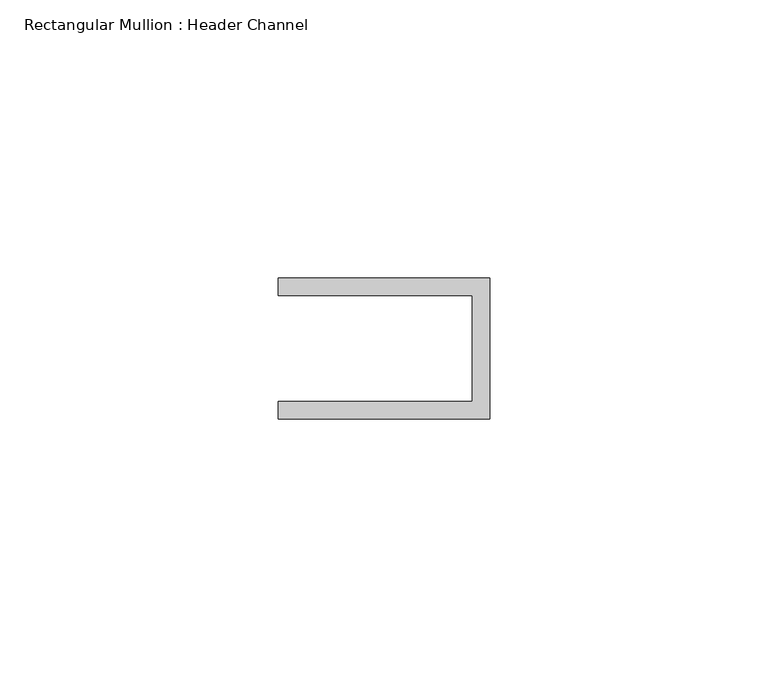
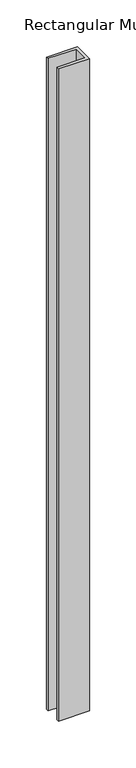
"""IFC4 building model written with IfcOpenShell, lengths in millimetres: member geometry, Rectangular Mullion : Header Channel."""

from ifc_helpers import new_model, si_unit, frame, origin, place, context, project, spatial, polyline, outline, extrude, source, transform, mapped, element, save


def rectangular_mullion_header_channel_4acfc972(model_context):
    return source(origin(), model_context, "Body", "SweptSolid", [
        extrude(outline(polyline([(0.0, -12.7), (-38.1, -12.7), (-38.1, -9.525), (-3.175, -9.525), (-3.175, 9.525), (-38.1, 9.525), (-38.1, 12.7), (0.0, 12.7), (0.0, -12.7)])), frame((0.0, 0.0, -851.126786), z_axis=(0.0, 0.0, 1.0), x_axis=(1.0, 0.0, 0.0)), (0.0, 0.0, 1.0), 851.126786),
    ])


if __name__ == "__main__":
    model = new_model("IFC4")
    model_context = context("Model", 3, world=origin())
    ifc_project = project(units=[si_unit("LENGTHUNIT", "METRE", prefix="MILLI")], contexts=[model_context])
    site = spatial("IfcSite", under=ifc_project)
    building = spatial("IfcBuilding", under=site)
    placement = place(None, origin())
    rectangular_mullion_header_channel_shape = rectangular_mullion_header_channel_4acfc972(model_context)
    element("IfcMember", 1, ObjectType="Rectangular Mullion : Header Channel", at=placement, inside=building, context=model_context, shape_type="MappedRepresentation", body=[
        mapped(rectangular_mullion_header_channel_shape, transform((0.0, 0.0, 0.0), x_axis=(1.0, 0.0, 0.0), y_axis=(0.0, 1.0, 0.0), z_axis=(0.0, 0.0, 1.0))),
    ])
    save(model, "model.ifc")

# Revit data of these elements
# Type "Rectangular Mullion : Header Channel"
#   built-in parameter 1007322 = 0.0833333 (stored number, unit not read)
#   built-in parameter 1007321 = -0.03125 (stored number, unit not read)
#   built-in parameter 1007320 = 0.0416667 (stored number, unit not read)
# Element 1 (IfcMember, "Rectangular Mullion : Header Channel")
#   Materials on its faces: "ALUM"
# Materials
#   "ALUM": class "Generic", colour RGB 157 157 157, transparency 0, Cost = 0
